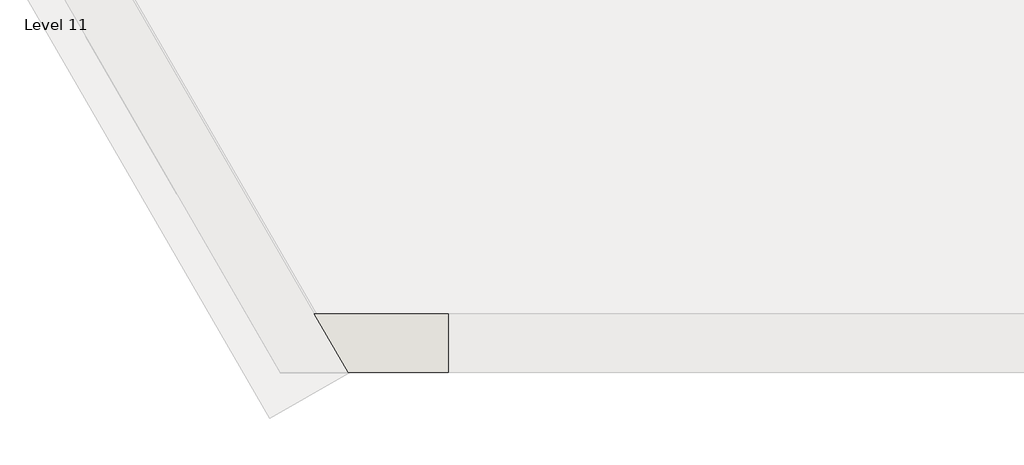
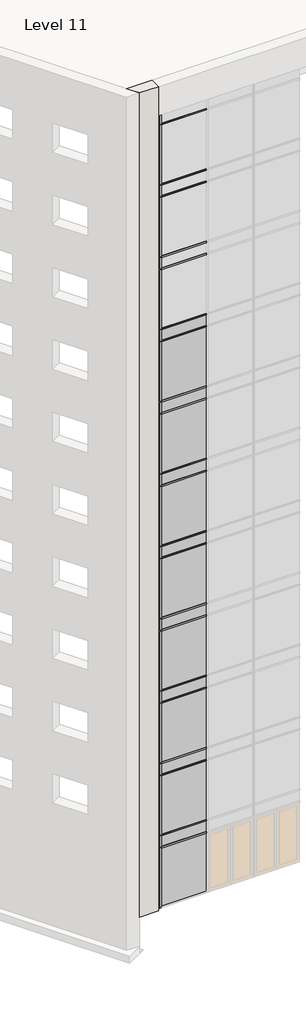
# One storey, part 1 of 6: 89 members, 38 plates, 1 wall.
"""IFC4 building model written with IfcOpenShell, lengths in millimetres."""

import ifcopenshell
import ifcopenshell.guid

model = None  # the IFC model being written
_history = None  # IfcOwnerHistory: only IFC2X3 demands one
_inside = {}  # id of a spatial element -> (the spatial element, [elements in it])
_under = {}  # id of a project, library or spatial element -> (it, [spatial elements below it])
_declared = {}  # id of a project -> (the project, [libraries it declares])
_typed = {}  # id of a type object -> (the type object, [elements of that type])
_made_of = {}  # id of a material, layer set ... -> (it, [elements and type objects made of it])


def new_model(schema):
    """Start an empty IFC model of exactly this schema.

    Asked for "IFC4X3", IfcOpenShell would pick the latest addendum, in which some entities
    have other attributes; the version numbers below select the first issue.
    IFC2X3 requires an IfcOwnerHistory on every rooted entity: one is made here for all.
    """
    global model, _history
    if schema == "IFC4X3":
        model = ifcopenshell.file(schema_version=(4, 3, 0, 0))
    else:
        model = ifcopenshell.file(schema=schema)
    _inside.clear()
    _under.clear()
    _declared.clear()
    _typed.clear()
    _made_of.clear()
    _history = None
    if model.schema == "IFC2X3":
        org = make("IfcOrganization", Name="unknown")
        user = make(
            "IfcPersonAndOrganization",
            ThePerson=make("IfcPerson", FamilyName="unknown"),
            TheOrganization=org,
        )
        app = make(
            "IfcApplication",
            ApplicationDeveloper=org,
            Version="unknown",
            ApplicationFullName="unknown",
            ApplicationIdentifier="unknown",
        )
        _history = make(
            "IfcOwnerHistory",
            OwningUser=user,
            OwningApplication=app,
            ChangeAction="ADDED",
            CreationDate=0,
        )
    return model


def make(cls, **values):
    """One entity of the class cls with the attributes given. An attribute that is None is left unset."""
    return model.create_entity(
        cls, **{name: value for name, value in values.items() if value is not None}
    )


def rooted(cls, **values):
    """An entity with a GlobalId (a new one), such as an element, a storey or a relation."""
    return make(cls, GlobalId=ifcopenshell.guid.new(), OwnerHistory=_history, **values)


def si_unit(unit_type, name, prefix=None):
    """IfcSIUnit, for example si_unit("LENGTHUNIT", "METRE", prefix="MILLI")."""
    return make("IfcSIUnit", UnitType=unit_type, Prefix=prefix, Name=name)


def assignment(units):
    """IfcUnitAssignment: the units of a project."""
    return None if units is None else make("IfcUnitAssignment", Units=units)


def point(xyz):
    """IfcCartesianPoint."""
    return None if xyz is None else make("IfcCartesianPoint", Coordinates=xyz)


def direction(xyz):
    """IfcDirection."""
    return None if xyz is None else make("IfcDirection", DirectionRatios=xyz)


def frame(location, z_axis=None, x_axis=None):
    """IfcAxis2Placement3D, a coordinate frame: its origin and axes. An axis left out is left unset."""
    return make(
        "IfcAxis2Placement3D",
        Location=point(location),
        Axis=direction(z_axis),
        RefDirection=direction(x_axis),
    )


def origin():
    """The frame at (0, 0, 0) with its axes left unset."""
    return frame((0.0, 0.0, 0.0))


def origin_with_axes():
    """The frame at (0, 0, 0) with the z axis (0, 0, 1) and the x axis (1, 0, 0) written out."""
    return frame((0.0, 0.0, 0.0), z_axis=(0.0, 0.0, 1.0), x_axis=(1.0, 0.0, 0.0))


def place(relative_to, where):
    """IfcLocalPlacement: puts the frame where relative to a parent placement (None: the world)."""
    return make(
        "IfcLocalPlacement", PlacementRelTo=relative_to, RelativePlacement=where
    )


def context(
    kind, dimensions, precision=None, world=None, true_north=None, identifier=None
):
    """IfcGeometricRepresentationContext, for example the 3D "Model" context."""
    return make(
        "IfcGeometricRepresentationContext",
        ContextIdentifier=identifier,
        ContextType=kind,
        CoordinateSpaceDimension=dimensions,
        Precision=precision,
        WorldCoordinateSystem=world,
        TrueNorth=true_north,
    )


def project(units=None, contexts=None):
    """IfcProject with its units and contexts."""
    return rooted(
        "IfcProject",
        Name="project",
        RepresentationContexts=contexts,
        UnitsInContext=assignment(units),
    )


def spatial(cls, under=None, at=None, **own):
    """A site, building, storey or space (cls), placed at a placement, below another one or the project."""
    s = rooted(cls, ObjectPlacement=at, **own)
    if under is not None:
        _under.setdefault(under.id(), (under, []))[1].append(s)
    return s


def polyline(points):
    """IfcPolyline through the points."""
    return make("IfcPolyline", Points=[point(p) for p in points])


def outline(outer, holes=None, kind="AREA"):
    """IfcArbitraryClosedProfileDef: a profile drawn as a closed curve; with holes, ...WithVoids."""
    if holes is None:
        return make("IfcArbitraryClosedProfileDef", ProfileType=kind, OuterCurve=outer)
    return make(
        "IfcArbitraryProfileDefWithVoids",
        ProfileType=kind,
        OuterCurve=outer,
        InnerCurves=holes,
    )


def extrude(swept, where, along, depth):
    """IfcExtrudedAreaSolid: the profile swept, set in the frame where, extruded along a direction by depth."""
    return make(
        "IfcExtrudedAreaSolid",
        SweptArea=swept,
        Position=where,
        ExtrudedDirection=direction(along),
        Depth=depth,
    )


def shape(context_of_items, identifier, shape_type, items):
    """IfcShapeRepresentation: the items that make up one representation, for example the "Body"."""
    return make(
        "IfcShapeRepresentation",
        ContextOfItems=context_of_items,
        RepresentationIdentifier=identifier,
        RepresentationType=shape_type,
        Items=items,
    )


def source(mapping_origin, context_of_items, identifier, shape_type, items):
    """IfcRepresentationMap: a shape defined once, which mapped items show again and again."""
    return make(
        "IfcRepresentationMap",
        MappingOrigin=mapping_origin,
        MappedRepresentation=shape(context_of_items, identifier, shape_type, items),
    )


def transform(
    local_origin,
    x_axis=None,
    y_axis=None,
    z_axis=None,
    scale=None,
    scale2=None,
    scale3=None,
    uniform=True,
):
    """IfcCartesianTransformationOperator3D, or its non-uniform kind. x_axis, y_axis, z_axis: its Axis1, 2, 3."""
    if uniform:
        return make(
            "IfcCartesianTransformationOperator3D",
            Axis1=direction(x_axis),
            Axis2=direction(y_axis),
            LocalOrigin=point(local_origin),
            Scale=scale,
            Axis3=direction(z_axis),
        )
    return make(
        "IfcCartesianTransformationOperator3DnonUniform",
        Axis1=direction(x_axis),
        Axis2=direction(y_axis),
        LocalOrigin=point(local_origin),
        Scale=scale,
        Axis3=direction(z_axis),
        Scale2=scale2,
        Scale3=scale3,
    )


def mapped(mapping_source, mapping_target):
    """IfcMappedItem: shows the shape of a source again, moved by a transform."""
    return make(
        "IfcMappedItem", MappingSource=mapping_source, MappingTarget=mapping_target
    )


def made_of(thing, what):
    """Note that an element or type object is made of a material, layer set ...; save() writes the relation."""
    if what is not None:
        _made_of.setdefault(what.id(), (what, []))[1].append(thing)
    return thing


def element(
    cls,
    number,
    at=None,
    inside=None,
    cuts=None,
    type_object=None,
    material=None,
    context=None,
    identifier="Body",
    shape_type=None,
    held_by="IfcProductDefinitionShape",
    body=None,
    shapes=None,
    **own,
):
    """One element of the class cls, such as IfcWall. Its Tag is "e" and its number.

    at: its placement. inside: the storey or other place that contains it. cuts: it is an
    opening in that element (IfcRelVoidsElement). A single representation is given by context,
    identifier, shape_type and body (its items); several are given by shapes. held_by: the class
    of the entity that holds the representations. save() writes the other relations.
    """
    e = rooted(cls, Tag="e%d" % number, ObjectPlacement=at, **own)
    if body is not None:
        shapes = [shape(context, identifier, shape_type, body)]
    if shapes is not None:
        e.Representation = make(held_by, Representations=shapes)
    if inside is not None:
        _inside.setdefault(inside.id(), (inside, []))[1].append(e)
    if cuts is not None:
        rooted(
            "IfcRelVoidsElement", RelatingBuildingElement=cuts, RelatedOpeningElement=e
        )
    if type_object is not None:
        _typed.setdefault(type_object.id(), (type_object, []))[1].append(e)
    return made_of(e, material)


def aggregate(whole, parts):
    """IfcRelAggregates: a whole, such as a stair, and the parts it consists of."""
    return rooted("IfcRelAggregates", RelatingObject=whole, RelatedObjects=parts)


def save(model, path):
    """Write the relations noted so far, then the file.

    IfcRelAggregates (storeys below a building ...), IfcRelContainedInSpatialStructure (elements
    in a storey), IfcRelDefinesByType, IfcRelAssociatesMaterial and IfcRelDeclares: one each for
    every whole, place, type object, material and project.
    """
    for whole, parts in _under.values():
        aggregate(whole, parts)
    for where, things in _inside.values():
        rooted(
            "IfcRelContainedInSpatialStructure",
            RelatedElements=things,
            RelatingStructure=where,
        )
    for kind, things in _typed.values():
        rooted("IfcRelDefinesByType", RelatedObjects=things, RelatingType=kind)
    for what, things in _made_of.values():
        rooted("IfcRelAssociatesMaterial", RelatedObjects=things, RelatingMaterial=what)
    for by, libraries in _declared.values():
        rooted("IfcRelDeclares", RelatingContext=by, RelatedDefinitions=libraries)
    model.write(path)


def rectangular_mullion_50x150mm_eb9201c3(model_context):
    return source(origin(), model_context, "Body", "SweptSolid", [
        extrude(outline(polyline([(25.0, 75.0), (25.0, -75.0), (-25.0, -75.0), (-25.0, 75.0), (25.0, 75.0)])), frame((0.0, 0.0, -2500.0), z_axis=(0.0, 0.0, 1.0), x_axis=(1.0, 0.0, 0.0)), (0.0, 0.0, 1.0), 2500.0),
    ])


def rectangular_mullion_50x150mm_f5b8645b(model_context):
    return source(origin(), model_context, "Body", "SweptSolid", [
        extrude(outline(polyline([(25.0, 75.0), (25.0, -75.0), (-25.0, -75.0), (-25.0, 75.0), (25.0, 75.0)])), frame((0.0, 0.0, -1780.0), z_axis=(0.0, 0.0, 1.0), x_axis=(1.0, 0.0, 0.0)), (0.0, 0.0, 1.0), 1780.0),
    ])


def rectangular_mullion_50x150mm_ded00a16(model_context):
    return source(origin(), model_context, "Body", "SweptSolid", [
        extrude(outline(polyline([(0.0, 75.0), (0.0, -75.0), (-50.0, -75.0), (-50.0, 75.0), (0.0, 75.0)])), frame((0.0, 0.0, -1780.0), z_axis=(0.0, 0.0, 1.0), x_axis=(1.0, 0.0, 0.0)), (0.0, 0.0, 1.0), 1780.0),
    ])


def rectangular_mullion_50x150mm_22f77a7a(model_context):
    return source(origin(), model_context, "Body", "SweptSolid", [
        extrude(outline(polyline([(25.0, 75.0), (25.0, -75.0), (-25.0, -75.0), (-25.0, 75.0), (25.0, 75.0)])), frame((0.0, 0.0, -500.0), z_axis=(0.0, 0.0, 1.0), x_axis=(1.0, 0.0, 0.0)), (0.0, 0.0, 1.0), 500.0),
    ])


def rectangular_mullion_50x150mm_4c3b9bdb(model_context):
    return source(origin(), model_context, "Body", "SweptSolid", [
        extrude(outline(polyline([(0.0, 75.0), (0.0, -75.0), (-50.0, -75.0), (-50.0, 75.0), (0.0, 75.0)])), frame((0.0, 0.0, -2500.0), z_axis=(0.0, 0.0, 1.0), x_axis=(1.0, 0.0, 0.0)), (0.0, 0.0, 1.0), 2500.0),
    ])


def rectangular_mullion_50x150mm_b3666dbd(model_context):
    return source(origin(), model_context, "Body", "SweptSolid", [
        extrude(outline(polyline([(0.0, 75.0), (0.0, -75.0), (-50.0, -75.0), (-50.0, 75.0), (0.0, 75.0)])), frame((0.0, 0.0, -500.0), z_axis=(0.0, 0.0, 1.0), x_axis=(1.0, 0.0, 0.0)), (0.0, 0.0, 1.0), 500.0),
    ])


def rectangular_mullion_50x150mm_6eefbde0(model_context):
    return source(origin(), model_context, "Body", "SweptSolid", [
        extrude(outline(polyline([(0.0, 75.0), (0.0, -75.0), (-50.0, -75.0), (-50.0, 75.0), (0.0, 75.0)])), frame((0.0, 0.0, -74.4185145), z_axis=(0.0, 0.0, 1.0), x_axis=(1.0, 0.0, 0.0)), (0.0, 0.0, 1.0), 74.4185145),
    ])


def rectangular_mullion_50x150mm_0166ad73(model_context):
    return source(origin(), model_context, "Body", "SweptSolid", [
        extrude(outline(polyline([(25.0, 75.0), (25.0, -75.0), (-25.0, -75.0), (-25.0, 75.0), (25.0, 75.0)])), frame((0.0, 0.0, -74.4185145), z_axis=(0.0, 0.0, 1.0), x_axis=(1.0, 0.0, 0.0)), (0.0, 0.0, 1.0), 74.4185145),
    ])


def system_panel_glazed_37b58b52(model_context):
    return source(origin(), model_context, "Body", "SweptSolid", [
        extrude(outline(polyline([(890.0, 24.5), (-890.0, 24.5), (-890.0, 49.5), (890.0, 49.5), (890.0, 24.5)])), origin_with_axes(), (0.0, 0.0, 1.0), 2425.0),
    ])


def system_panel_glazed_87c86ac8(model_context):
    return source(origin(), model_context, "Body", "SweptSolid", [
        extrude(outline(polyline([(890.0, 24.5), (-890.0, 24.5), (-890.0, 49.5), (890.0, 49.5), (890.0, 24.5)])), origin_with_axes(), (0.0, 0.0, 1.0), 450.0),
    ])


def system_panel_glazed_3dade0f0(model_context):
    return source(origin(), model_context, "Body", "SweptSolid", [
        extrude(outline(polyline([(890.0, 24.5), (-890.0, 24.5), (-890.0, 49.5), (890.0, 49.5), (890.0, 24.5)])), origin_with_axes(), (0.0, 0.0, 1.0), 2450.0),
    ])


def system_panel_glazed_e32ff5c7(model_context):
    return source(origin(), model_context, "Body", "SweptSolid", [
        extrude(outline(polyline([(37.2092572, 24.5), (-37.2092572, 24.5), (-37.2092572, 49.5), (37.2092572, 49.5), (37.2092572, 24.5)])), origin_with_axes(), (0.0, 0.0, 1.0), 2425.0),
    ])


def system_panel_glazed_b42e89e7(model_context):
    return source(origin(), model_context, "Body", "SweptSolid", [
        extrude(outline(polyline([(37.2092572, 24.5), (-37.2092572, 24.5), (-37.2092572, 49.5), (37.2092572, 49.5), (37.2092572, 24.5)])), origin_with_axes(), (0.0, 0.0, 1.0), 450.0),
    ])


def system_panel_glazed_54eb7814(model_context):
    return source(origin(), model_context, "Body", "SweptSolid", [
        extrude(outline(polyline([(37.2092572, 24.5), (-37.2092572, 24.5), (-37.2092572, 49.5), (37.2092572, 49.5), (37.2092572, 24.5)])), origin_with_axes(), (0.0, 0.0, 1.0), 2450.0),
    ])


def system_panel_glazed_e987ce54(model_context):
    return source(origin(), model_context, "Body", "SweptSolid", [
        extrude(outline(polyline([(37.2092572, 24.5), (-37.2092572, 24.5), (-37.2092572, 49.5), (37.2092572, 49.5), (37.2092572, 24.5)])), origin_with_axes(), (0.0, 0.0, 1.0), 425.0),
    ])


model = new_model("IFC4")

# Units and contexts
model_context = context("Model", 3, world=origin())
ifc_project = project(units=[si_unit("LENGTHUNIT", "METRE", prefix="MILLI")], contexts=[model_context])

# Site, building, storey
site = spatial("IfcSite", under=ifc_project)
building = spatial("IfcBuilding", under=site)
storey = spatial("IfcBuildingStorey", under=building, Name="Level 11", Elevation=33000.0)

# Members
placement = place(None, origin())
rectangular_mullion_50x150mm_shape = rectangular_mullion_50x150mm_eb9201c3(model_context)
element("IfcMember", 1, ObjectType="Rectangular Mullion : 50x150mm", at=placement, inside=storey, context=model_context, shape_type="MappedRepresentation", body=[
    mapped(rectangular_mullion_50x150mm_shape, transform((-3631.4360441, -8316.0631989, 0.0), x_axis=(-1.0, 0.0, 0.0), y_axis=(0.0, 1.0, 0.0), z_axis=(0.0, 0.0, -1.0))),
])
rectangular_mullion_50x150mm_2_shape = rectangular_mullion_50x150mm_f5b8645b(model_context)
element("IfcMember", 2, ObjectType="Rectangular Mullion : 50x150mm", at=placement, inside=storey, context=model_context, shape_type="MappedRepresentation", body=[
    mapped(rectangular_mullion_50x150mm_2_shape, transform((-3606.4360441, -8316.0631989, 2500.0), x_axis=(0.0, 0.0, 1.0), y_axis=(0.0, 1.0, 0.0), z_axis=(-1.0, 0.0, 0.0))),
])
element("IfcMember", 3, ObjectType="Rectangular Mullion : 50x150mm", at=placement, inside=storey, context=model_context, shape_type="MappedRepresentation", body=[
    mapped(rectangular_mullion_50x150mm_2_shape, transform((-3606.4360441, -8316.0631989, 5500.0), x_axis=(0.0, 0.0, 1.0), y_axis=(0.0, 1.0, 0.0), z_axis=(-1.0, 0.0, 0.0))),
])
element("IfcMember", 4, ObjectType="Rectangular Mullion : 50x150mm", at=placement, inside=storey, context=model_context, shape_type="MappedRepresentation", body=[
    mapped(rectangular_mullion_50x150mm_2_shape, transform((-3606.4360441, -8316.0631989, 8500.0), x_axis=(0.0, 0.0, 1.0), y_axis=(0.0, 1.0, 0.0), z_axis=(-1.0, 0.0, 0.0))),
])
element("IfcMember", 5, ObjectType="Rectangular Mullion : 50x150mm", at=placement, inside=storey, context=model_context, shape_type="MappedRepresentation", body=[
    mapped(rectangular_mullion_50x150mm_2_shape, transform((-3606.4360441, -8316.0631989, 11500.0), x_axis=(0.0, 0.0, 1.0), y_axis=(0.0, 1.0, 0.0), z_axis=(-1.0, 0.0, 0.0))),
])
element("IfcMember", 6, ObjectType="Rectangular Mullion : 50x150mm", at=placement, inside=storey, context=model_context, shape_type="MappedRepresentation", body=[
    mapped(rectangular_mullion_50x150mm_2_shape, transform((-3606.4360441, -8316.0631989, 14500.0), x_axis=(0.0, 0.0, 1.0), y_axis=(0.0, 1.0, 0.0), z_axis=(-1.0, 0.0, 0.0))),
])
element("IfcMember", 7, ObjectType="Rectangular Mullion : 50x150mm", at=placement, inside=storey, context=model_context, shape_type="MappedRepresentation", body=[
    mapped(rectangular_mullion_50x150mm_2_shape, transform((-3606.4360441, -8316.0631989, 17500.0), x_axis=(0.0, 0.0, 1.0), y_axis=(0.0, 1.0, 0.0), z_axis=(-1.0, 0.0, 0.0))),
])
element("IfcMember", 8, ObjectType="Rectangular Mullion : 50x150mm", at=placement, inside=storey, context=model_context, shape_type="MappedRepresentation", body=[
    mapped(rectangular_mullion_50x150mm_2_shape, transform((-3606.4360441, -8316.0631989, 20500.0), x_axis=(0.0, 0.0, 1.0), y_axis=(0.0, 1.0, 0.0), z_axis=(-1.0, 0.0, 0.0))),
])
element("IfcMember", 9, ObjectType="Rectangular Mullion : 50x150mm", at=placement, inside=storey, context=model_context, shape_type="MappedRepresentation", body=[
    mapped(rectangular_mullion_50x150mm_2_shape, transform((-3606.4360441, -8316.0631989, 23500.0), x_axis=(0.0, 0.0, 1.0), y_axis=(0.0, 1.0, 0.0), z_axis=(-1.0, 0.0, 0.0))),
])
element("IfcMember", 10, ObjectType="Rectangular Mullion : 50x150mm", at=placement, inside=storey, context=model_context, shape_type="MappedRepresentation", body=[
    mapped(rectangular_mullion_50x150mm_2_shape, transform((-3606.4360441, -8316.0631989, 3000.0), x_axis=(0.0, 0.0, 1.0), y_axis=(0.0, 1.0, 0.0), z_axis=(-1.0, 0.0, 0.0))),
])
element("IfcMember", 11, ObjectType="Rectangular Mullion : 50x150mm", at=placement, inside=storey, context=model_context, shape_type="MappedRepresentation", body=[
    mapped(rectangular_mullion_50x150mm_2_shape, transform((-3606.4360441, -8316.0631989, 6000.0), x_axis=(0.0, 0.0, 1.0), y_axis=(0.0, 1.0, 0.0), z_axis=(-1.0, 0.0, 0.0))),
])
element("IfcMember", 12, ObjectType="Rectangular Mullion : 50x150mm", at=placement, inside=storey, context=model_context, shape_type="MappedRepresentation", body=[
    mapped(rectangular_mullion_50x150mm_2_shape, transform((-3606.4360441, -8316.0631989, 9000.0), x_axis=(0.0, 0.0, 1.0), y_axis=(0.0, 1.0, 0.0), z_axis=(-1.0, 0.0, 0.0))),
])
element("IfcMember", 13, ObjectType="Rectangular Mullion : 50x150mm", at=placement, inside=storey, context=model_context, shape_type="MappedRepresentation", body=[
    mapped(rectangular_mullion_50x150mm_2_shape, transform((-3606.4360441, -8316.0631989, 12000.0), x_axis=(0.0, 0.0, 1.0), y_axis=(0.0, 1.0, 0.0), z_axis=(-1.0, 0.0, 0.0))),
])
element("IfcMember", 14, ObjectType="Rectangular Mullion : 50x150mm", at=placement, inside=storey, context=model_context, shape_type="MappedRepresentation", body=[
    mapped(rectangular_mullion_50x150mm_2_shape, transform((-3606.4360441, -8316.0631989, 15000.0), x_axis=(0.0, 0.0, 1.0), y_axis=(0.0, 1.0, 0.0), z_axis=(-1.0, 0.0, 0.0))),
])
element("IfcMember", 15, ObjectType="Rectangular Mullion : 50x150mm", at=placement, inside=storey, context=model_context, shape_type="MappedRepresentation", body=[
    mapped(rectangular_mullion_50x150mm_2_shape, transform((-3606.4360441, -8316.0631989, 18000.0), x_axis=(0.0, 0.0, 1.0), y_axis=(0.0, 1.0, 0.0), z_axis=(-1.0, 0.0, 0.0))),
])
element("IfcMember", 16, ObjectType="Rectangular Mullion : 50x150mm", at=placement, inside=storey, context=model_context, shape_type="MappedRepresentation", body=[
    mapped(rectangular_mullion_50x150mm_2_shape, transform((-3606.4360441, -8316.0631989, 21000.0), x_axis=(0.0, 0.0, 1.0), y_axis=(0.0, 1.0, 0.0), z_axis=(-1.0, 0.0, 0.0))),
])
element("IfcMember", 17, ObjectType="Rectangular Mullion : 50x150mm", at=placement, inside=storey, context=model_context, shape_type="MappedRepresentation", body=[
    mapped(rectangular_mullion_50x150mm_2_shape, transform((-3606.4360441, -8316.0631989, 24000.0), x_axis=(0.0, 0.0, 1.0), y_axis=(0.0, 1.0, 0.0), z_axis=(-1.0, 0.0, 0.0))),
])
element("IfcMember", 18, ObjectType="Rectangular Mullion : 50x150mm", at=placement, inside=storey, context=model_context, shape_type="MappedRepresentation", body=[
    mapped(rectangular_mullion_50x150mm_2_shape, transform((-3606.4360441, -8316.0631989, 27000.0), x_axis=(0.0, 0.0, 1.0), y_axis=(0.0, 1.0, 0.0), z_axis=(-1.0, 0.0, 0.0))),
])
element("IfcMember", 19, ObjectType="Rectangular Mullion : 50x150mm", at=placement, inside=storey, context=model_context, shape_type="MappedRepresentation", body=[
    mapped(rectangular_mullion_50x150mm_2_shape, transform((-3606.4360441, -8316.0631989, 26500.0), x_axis=(0.0, 0.0, 1.0), y_axis=(0.0, 1.0, 0.0), z_axis=(-1.0, 0.0, 0.0))),
])
element("IfcMember", 20, ObjectType="Rectangular Mullion : 50x150mm", at=placement, inside=storey, context=model_context, shape_type="MappedRepresentation", body=[
    mapped(rectangular_mullion_50x150mm_2_shape, transform((-3606.4360441, -8316.0631989, 30000.0), x_axis=(0.0, 0.0, 1.0), y_axis=(0.0, 1.0, 0.0), z_axis=(-1.0, 0.0, 0.0))),
])
element("IfcMember", 21, ObjectType="Rectangular Mullion : 50x150mm", at=placement, inside=storey, context=model_context, shape_type="MappedRepresentation", body=[
    mapped(rectangular_mullion_50x150mm_2_shape, transform((-3606.4360441, -8316.0631989, 29500.0), x_axis=(0.0, 0.0, 1.0), y_axis=(0.0, 1.0, 0.0), z_axis=(-1.0, 0.0, 0.0))),
])
element("IfcMember", 22, ObjectType="Rectangular Mullion : 50x150mm", at=placement, inside=storey, context=model_context, shape_type="MappedRepresentation", body=[
    mapped(rectangular_mullion_50x150mm_2_shape, transform((-3606.4360441, -8316.0631989, 32500.0), x_axis=(0.0, 0.0, 1.0), y_axis=(0.0, 1.0, 0.0), z_axis=(-1.0, 0.0, 0.0))),
])
rectangular_mullion_50x150mm_3_shape = rectangular_mullion_50x150mm_ded00a16(model_context)
element("IfcMember", 23, ObjectType="Rectangular Mullion : 50x150mm", at=placement, inside=storey, context=model_context, shape_type="MappedRepresentation", body=[
    mapped(rectangular_mullion_50x150mm_3_shape, transform((-3606.4360441, -8316.0631989, 33000.0), x_axis=(0.0, 0.0, 1.0), y_axis=(0.0, 1.0, 0.0), z_axis=(-1.0, 0.0, 0.0))),
])
rectangular_mullion_50x150mm_4_shape = rectangular_mullion_50x150mm_22f77a7a(model_context)
element("IfcMember", 24, ObjectType="Rectangular Mullion : 50x150mm", at=placement, inside=storey, context=model_context, shape_type="MappedRepresentation", body=[
    mapped(rectangular_mullion_50x150mm_4_shape, transform((-3631.4360441, -8316.0631989, 2500.0), x_axis=(-1.0, 0.0, 0.0), y_axis=(0.0, 1.0, 0.0), z_axis=(0.0, 0.0, -1.0))),
])
element("IfcMember", 25, ObjectType="Rectangular Mullion : 50x150mm", at=placement, inside=storey, context=model_context, shape_type="MappedRepresentation", body=[
    mapped(rectangular_mullion_50x150mm_4_shape, transform((-3631.4360441, -8316.0631989, 5500.0), x_axis=(-1.0, 0.0, 0.0), y_axis=(0.0, 1.0, 0.0), z_axis=(0.0, 0.0, -1.0))),
])
element("IfcMember", 26, ObjectType="Rectangular Mullion : 50x150mm", at=placement, inside=storey, context=model_context, shape_type="MappedRepresentation", body=[
    mapped(rectangular_mullion_50x150mm_4_shape, transform((-3631.4360441, -8316.0631989, 8500.0), x_axis=(-1.0, 0.0, 0.0), y_axis=(0.0, 1.0, 0.0), z_axis=(0.0, 0.0, -1.0))),
])
element("IfcMember", 27, ObjectType="Rectangular Mullion : 50x150mm", at=placement, inside=storey, context=model_context, shape_type="MappedRepresentation", body=[
    mapped(rectangular_mullion_50x150mm_4_shape, transform((-3631.4360441, -8316.0631989, 11500.0), x_axis=(-1.0, 0.0, 0.0), y_axis=(0.0, 1.0, 0.0), z_axis=(0.0, 0.0, -1.0))),
])
element("IfcMember", 28, ObjectType="Rectangular Mullion : 50x150mm", at=placement, inside=storey, context=model_context, shape_type="MappedRepresentation", body=[
    mapped(rectangular_mullion_50x150mm_4_shape, transform((-3631.4360441, -8316.0631989, 14500.0), x_axis=(-1.0, 0.0, 0.0), y_axis=(0.0, 1.0, 0.0), z_axis=(0.0, 0.0, -1.0))),
])
element("IfcMember", 29, ObjectType="Rectangular Mullion : 50x150mm", at=placement, inside=storey, context=model_context, shape_type="MappedRepresentation", body=[
    mapped(rectangular_mullion_50x150mm_4_shape, transform((-3631.4360441, -8316.0631989, 17500.0), x_axis=(-1.0, 0.0, 0.0), y_axis=(0.0, 1.0, 0.0), z_axis=(0.0, 0.0, -1.0))),
])
element("IfcMember", 30, ObjectType="Rectangular Mullion : 50x150mm", at=placement, inside=storey, context=model_context, shape_type="MappedRepresentation", body=[
    mapped(rectangular_mullion_50x150mm_4_shape, transform((-3631.4360441, -8316.0631989, 20500.0), x_axis=(-1.0, 0.0, 0.0), y_axis=(0.0, 1.0, 0.0), z_axis=(0.0, 0.0, -1.0))),
])
element("IfcMember", 31, ObjectType="Rectangular Mullion : 50x150mm", at=placement, inside=storey, context=model_context, shape_type="MappedRepresentation", body=[
    mapped(rectangular_mullion_50x150mm_4_shape, transform((-3631.4360441, -8316.0631989, 23500.0), x_axis=(-1.0, 0.0, 0.0), y_axis=(0.0, 1.0, 0.0), z_axis=(0.0, 0.0, -1.0))),
])
element("IfcMember", 32, ObjectType="Rectangular Mullion : 50x150mm", at=placement, inside=storey, context=model_context, shape_type="MappedRepresentation", body=[
    mapped(rectangular_mullion_50x150mm_4_shape, transform((-3631.4360441, -8316.0631989, 26500.0), x_axis=(-1.0, 0.0, 0.0), y_axis=(0.0, 1.0, 0.0), z_axis=(0.0, 0.0, -1.0))),
])
element("IfcMember", 33, ObjectType="Rectangular Mullion : 50x150mm", at=placement, inside=storey, context=model_context, shape_type="MappedRepresentation", body=[
    mapped(rectangular_mullion_50x150mm_4_shape, transform((-3631.4360441, -8316.0631989, 29500.0), x_axis=(-1.0, 0.0, 0.0), y_axis=(0.0, 1.0, 0.0), z_axis=(0.0, 0.0, -1.0))),
])
element("IfcMember", 34, ObjectType="Rectangular Mullion : 50x150mm", at=placement, inside=storey, context=model_context, shape_type="MappedRepresentation", body=[
    mapped(rectangular_mullion_50x150mm_shape, transform((-3631.4360441, -8316.0631989, 3000.0), x_axis=(-1.0, 0.0, 0.0), y_axis=(0.0, 1.0, 0.0), z_axis=(0.0, 0.0, -1.0))),
])
element("IfcMember", 35, ObjectType="Rectangular Mullion : 50x150mm", at=placement, inside=storey, context=model_context, shape_type="MappedRepresentation", body=[
    mapped(rectangular_mullion_50x150mm_shape, transform((-3631.4360441, -8316.0631989, 6000.0), x_axis=(-1.0, 0.0, 0.0), y_axis=(0.0, 1.0, 0.0), z_axis=(0.0, 0.0, -1.0))),
])
element("IfcMember", 36, ObjectType="Rectangular Mullion : 50x150mm", at=placement, inside=storey, context=model_context, shape_type="MappedRepresentation", body=[
    mapped(rectangular_mullion_50x150mm_shape, transform((-3631.4360441, -8316.0631989, 9000.0), x_axis=(-1.0, 0.0, 0.0), y_axis=(0.0, 1.0, 0.0), z_axis=(0.0, 0.0, -1.0))),
])
element("IfcMember", 37, ObjectType="Rectangular Mullion : 50x150mm", at=placement, inside=storey, context=model_context, shape_type="MappedRepresentation", body=[
    mapped(rectangular_mullion_50x150mm_shape, transform((-3631.4360441, -8316.0631989, 12000.0), x_axis=(-1.0, 0.0, 0.0), y_axis=(0.0, 1.0, 0.0), z_axis=(0.0, 0.0, -1.0))),
])
element("IfcMember", 38, ObjectType="Rectangular Mullion : 50x150mm", at=placement, inside=storey, context=model_context, shape_type="MappedRepresentation", body=[
    mapped(rectangular_mullion_50x150mm_shape, transform((-3631.4360441, -8316.0631989, 15000.0), x_axis=(-1.0, 0.0, 0.0), y_axis=(0.0, 1.0, 0.0), z_axis=(0.0, 0.0, -1.0))),
])
element("IfcMember", 39, ObjectType="Rectangular Mullion : 50x150mm", at=placement, inside=storey, context=model_context, shape_type="MappedRepresentation", body=[
    mapped(rectangular_mullion_50x150mm_shape, transform((-3631.4360441, -8316.0631989, 18000.0), x_axis=(-1.0, 0.0, 0.0), y_axis=(0.0, 1.0, 0.0), z_axis=(0.0, 0.0, -1.0))),
])
element("IfcMember", 40, ObjectType="Rectangular Mullion : 50x150mm", at=placement, inside=storey, context=model_context, shape_type="MappedRepresentation", body=[
    mapped(rectangular_mullion_50x150mm_shape, transform((-3631.4360441, -8316.0631989, 21000.0), x_axis=(-1.0, 0.0, 0.0), y_axis=(0.0, 1.0, 0.0), z_axis=(0.0, 0.0, -1.0))),
])
element("IfcMember", 41, ObjectType="Rectangular Mullion : 50x150mm", at=placement, inside=storey, context=model_context, shape_type="MappedRepresentation", body=[
    mapped(rectangular_mullion_50x150mm_shape, transform((-3631.4360441, -8316.0631989, 24000.0), x_axis=(-1.0, 0.0, 0.0), y_axis=(0.0, 1.0, 0.0), z_axis=(0.0, 0.0, -1.0))),
])
element("IfcMember", 42, ObjectType="Rectangular Mullion : 50x150mm", at=placement, inside=storey, context=model_context, shape_type="MappedRepresentation", body=[
    mapped(rectangular_mullion_50x150mm_shape, transform((-3631.4360441, -8316.0631989, 27000.0), x_axis=(-1.0, 0.0, 0.0), y_axis=(0.0, 1.0, 0.0), z_axis=(0.0, 0.0, -1.0))),
])
element("IfcMember", 43, ObjectType="Rectangular Mullion : 50x150mm", at=placement, inside=storey, context=model_context, shape_type="MappedRepresentation", body=[
    mapped(rectangular_mullion_50x150mm_shape, transform((-3631.4360441, -8316.0631989, 30000.0), x_axis=(-1.0, 0.0, 0.0), y_axis=(0.0, 1.0, 0.0), z_axis=(0.0, 0.0, -1.0))),
])
element("IfcMember", 44, ObjectType="Rectangular Mullion : 50x150mm", at=placement, inside=storey, context=model_context, shape_type="MappedRepresentation", body=[
    mapped(rectangular_mullion_50x150mm_4_shape, transform((-3631.4360441, -8316.0631989, 32500.0), x_axis=(-1.0, 0.0, 0.0), y_axis=(0.0, 1.0, 0.0), z_axis=(0.0, 0.0, -1.0))),
])
rectangular_mullion_50x150mm_5_shape = rectangular_mullion_50x150mm_4c3b9bdb(model_context)
element("IfcMember", 45, ObjectType="Rectangular Mullion : 50x150mm", at=placement, inside=storey, context=model_context, shape_type="MappedRepresentation", body=[
    mapped(rectangular_mullion_50x150mm_5_shape, transform((-3780.8545586, -8316.0631989, 0.0), x_axis=(-1.0, 0.0, 0.0), y_axis=(0.0, 1.0, 0.0), z_axis=(0.0, 0.0, -1.0))),
])
rectangular_mullion_50x150mm_6_shape = rectangular_mullion_50x150mm_b3666dbd(model_context)
element("IfcMember", 46, ObjectType="Rectangular Mullion : 50x150mm", at=placement, inside=storey, context=model_context, shape_type="MappedRepresentation", body=[
    mapped(rectangular_mullion_50x150mm_6_shape, transform((-3780.8545586, -8316.0631989, 2500.0), x_axis=(-1.0, 0.0, 0.0), y_axis=(0.0, 1.0, 0.0), z_axis=(0.0, 0.0, -1.0))),
])
element("IfcMember", 47, ObjectType="Rectangular Mullion : 50x150mm", at=placement, inside=storey, context=model_context, shape_type="MappedRepresentation", body=[
    mapped(rectangular_mullion_50x150mm_6_shape, transform((-3780.8545586, -8316.0631989, 5500.0), x_axis=(-1.0, 0.0, 0.0), y_axis=(0.0, 1.0, 0.0), z_axis=(0.0, 0.0, -1.0))),
])
element("IfcMember", 48, ObjectType="Rectangular Mullion : 50x150mm", at=placement, inside=storey, context=model_context, shape_type="MappedRepresentation", body=[
    mapped(rectangular_mullion_50x150mm_6_shape, transform((-3780.8545586, -8316.0631989, 8500.0), x_axis=(-1.0, 0.0, 0.0), y_axis=(0.0, 1.0, 0.0), z_axis=(0.0, 0.0, -1.0))),
])
element("IfcMember", 49, ObjectType="Rectangular Mullion : 50x150mm", at=placement, inside=storey, context=model_context, shape_type="MappedRepresentation", body=[
    mapped(rectangular_mullion_50x150mm_6_shape, transform((-3780.8545586, -8316.0631989, 11500.0), x_axis=(-1.0, 0.0, 0.0), y_axis=(0.0, 1.0, 0.0), z_axis=(0.0, 0.0, -1.0))),
])
element("IfcMember", 50, ObjectType="Rectangular Mullion : 50x150mm", at=placement, inside=storey, context=model_context, shape_type="MappedRepresentation", body=[
    mapped(rectangular_mullion_50x150mm_6_shape, transform((-3780.8545586, -8316.0631989, 14500.0), x_axis=(-1.0, 0.0, 0.0), y_axis=(0.0, 1.0, 0.0), z_axis=(0.0, 0.0, -1.0))),
])
element("IfcMember", 51, ObjectType="Rectangular Mullion : 50x150mm", at=placement, inside=storey, context=model_context, shape_type="MappedRepresentation", body=[
    mapped(rectangular_mullion_50x150mm_6_shape, transform((-3780.8545586, -8316.0631989, 17500.0), x_axis=(-1.0, 0.0, 0.0), y_axis=(0.0, 1.0, 0.0), z_axis=(0.0, 0.0, -1.0))),
])
element("IfcMember", 52, ObjectType="Rectangular Mullion : 50x150mm", at=placement, inside=storey, context=model_context, shape_type="MappedRepresentation", body=[
    mapped(rectangular_mullion_50x150mm_6_shape, transform((-3780.8545586, -8316.0631989, 20500.0), x_axis=(-1.0, 0.0, 0.0), y_axis=(0.0, 1.0, 0.0), z_axis=(0.0, 0.0, -1.0))),
])
element("IfcMember", 53, ObjectType="Rectangular Mullion : 50x150mm", at=placement, inside=storey, context=model_context, shape_type="MappedRepresentation", body=[
    mapped(rectangular_mullion_50x150mm_6_shape, transform((-3780.8545586, -8316.0631989, 23500.0), x_axis=(-1.0, 0.0, 0.0), y_axis=(0.0, 1.0, 0.0), z_axis=(0.0, 0.0, -1.0))),
])
element("IfcMember", 54, ObjectType="Rectangular Mullion : 50x150mm", at=placement, inside=storey, context=model_context, shape_type="MappedRepresentation", body=[
    mapped(rectangular_mullion_50x150mm_6_shape, transform((-3780.8545586, -8316.0631989, 26500.0), x_axis=(-1.0, 0.0, 0.0), y_axis=(0.0, 1.0, 0.0), z_axis=(0.0, 0.0, -1.0))),
])
element("IfcMember", 55, ObjectType="Rectangular Mullion : 50x150mm", at=placement, inside=storey, context=model_context, shape_type="MappedRepresentation", body=[
    mapped(rectangular_mullion_50x150mm_6_shape, transform((-3780.8545586, -8316.0631989, 29500.0), x_axis=(-1.0, 0.0, 0.0), y_axis=(0.0, 1.0, 0.0), z_axis=(0.0, 0.0, -1.0))),
])
element("IfcMember", 56, ObjectType="Rectangular Mullion : 50x150mm", at=placement, inside=storey, context=model_context, shape_type="MappedRepresentation", body=[
    mapped(rectangular_mullion_50x150mm_5_shape, transform((-3780.8545586, -8316.0631989, 3000.0), x_axis=(-1.0, 0.0, 0.0), y_axis=(0.0, 1.0, 0.0), z_axis=(0.0, 0.0, -1.0))),
])
element("IfcMember", 57, ObjectType="Rectangular Mullion : 50x150mm", at=placement, inside=storey, context=model_context, shape_type="MappedRepresentation", body=[
    mapped(rectangular_mullion_50x150mm_5_shape, transform((-3780.8545586, -8316.0631989, 6000.0), x_axis=(-1.0, 0.0, 0.0), y_axis=(0.0, 1.0, 0.0), z_axis=(0.0, 0.0, -1.0))),
])
element("IfcMember", 58, ObjectType="Rectangular Mullion : 50x150mm", at=placement, inside=storey, context=model_context, shape_type="MappedRepresentation", body=[
    mapped(rectangular_mullion_50x150mm_5_shape, transform((-3780.8545586, -8316.0631989, 9000.0), x_axis=(-1.0, 0.0, 0.0), y_axis=(0.0, 1.0, 0.0), z_axis=(0.0, 0.0, -1.0))),
])
element("IfcMember", 59, ObjectType="Rectangular Mullion : 50x150mm", at=placement, inside=storey, context=model_context, shape_type="MappedRepresentation", body=[
    mapped(rectangular_mullion_50x150mm_5_shape, transform((-3780.8545586, -8316.0631989, 12000.0), x_axis=(-1.0, 0.0, 0.0), y_axis=(0.0, 1.0, 0.0), z_axis=(0.0, 0.0, -1.0))),
])
element("IfcMember", 60, ObjectType="Rectangular Mullion : 50x150mm", at=placement, inside=storey, context=model_context, shape_type="MappedRepresentation", body=[
    mapped(rectangular_mullion_50x150mm_5_shape, transform((-3780.8545586, -8316.0631989, 15000.0), x_axis=(-1.0, 0.0, 0.0), y_axis=(0.0, 1.0, 0.0), z_axis=(0.0, 0.0, -1.0))),
])
element("IfcMember", 61, ObjectType="Rectangular Mullion : 50x150mm", at=placement, inside=storey, context=model_context, shape_type="MappedRepresentation", body=[
    mapped(rectangular_mullion_50x150mm_5_shape, transform((-3780.8545586, -8316.0631989, 18000.0), x_axis=(-1.0, 0.0, 0.0), y_axis=(0.0, 1.0, 0.0), z_axis=(0.0, 0.0, -1.0))),
])
element("IfcMember", 62, ObjectType="Rectangular Mullion : 50x150mm", at=placement, inside=storey, context=model_context, shape_type="MappedRepresentation", body=[
    mapped(rectangular_mullion_50x150mm_5_shape, transform((-3780.8545586, -8316.0631989, 21000.0), x_axis=(-1.0, 0.0, 0.0), y_axis=(0.0, 1.0, 0.0), z_axis=(0.0, 0.0, -1.0))),
])
element("IfcMember", 63, ObjectType="Rectangular Mullion : 50x150mm", at=placement, inside=storey, context=model_context, shape_type="MappedRepresentation", body=[
    mapped(rectangular_mullion_50x150mm_5_shape, transform((-3780.8545586, -8316.0631989, 24000.0), x_axis=(-1.0, 0.0, 0.0), y_axis=(0.0, 1.0, 0.0), z_axis=(0.0, 0.0, -1.0))),
])
element("IfcMember", 64, ObjectType="Rectangular Mullion : 50x150mm", at=placement, inside=storey, context=model_context, shape_type="MappedRepresentation", body=[
    mapped(rectangular_mullion_50x150mm_5_shape, transform((-3780.8545586, -8316.0631989, 27000.0), x_axis=(-1.0, 0.0, 0.0), y_axis=(0.0, 1.0, 0.0), z_axis=(0.0, 0.0, -1.0))),
])
element("IfcMember", 65, ObjectType="Rectangular Mullion : 50x150mm", at=placement, inside=storey, context=model_context, shape_type="MappedRepresentation", body=[
    mapped(rectangular_mullion_50x150mm_5_shape, transform((-3780.8545586, -8316.0631989, 30000.0), x_axis=(-1.0, 0.0, 0.0), y_axis=(0.0, 1.0, 0.0), z_axis=(0.0, 0.0, -1.0))),
])
element("IfcMember", 66, ObjectType="Rectangular Mullion : 50x150mm", at=placement, inside=storey, context=model_context, shape_type="MappedRepresentation", body=[
    mapped(rectangular_mullion_50x150mm_6_shape, transform((-3780.8545586, -8316.0631989, 32500.0), x_axis=(-1.0, 0.0, 0.0), y_axis=(0.0, 1.0, 0.0), z_axis=(0.0, 0.0, -1.0))),
])
rectangular_mullion_50x150mm_7_shape = rectangular_mullion_50x150mm_6eefbde0(model_context)
element("IfcMember", 67, ObjectType="Rectangular Mullion : 50x150mm", at=placement, inside=storey, context=model_context, shape_type="MappedRepresentation", body=[
    mapped(rectangular_mullion_50x150mm_7_shape, transform((-3730.8545586, -8316.0631989, 33000.0), x_axis=(0.0, 0.0, 1.0), y_axis=(0.0, 1.0, 0.0), z_axis=(-1.0, 0.0, 0.0))),
])
rectangular_mullion_50x150mm_8_shape = rectangular_mullion_50x150mm_0166ad73(model_context)
element("IfcMember", 68, ObjectType="Rectangular Mullion : 50x150mm", at=placement, inside=storey, context=model_context, shape_type="MappedRepresentation", body=[
    mapped(rectangular_mullion_50x150mm_8_shape, transform((-3730.8545586, -8316.0631989, 2500.0), x_axis=(0.0, 0.0, 1.0), y_axis=(0.0, 1.0, 0.0), z_axis=(-1.0, 0.0, 0.0))),
])
element("IfcMember", 69, ObjectType="Rectangular Mullion : 50x150mm", at=placement, inside=storey, context=model_context, shape_type="MappedRepresentation", body=[
    mapped(rectangular_mullion_50x150mm_8_shape, transform((-3730.8545586, -8316.0631989, 5500.0), x_axis=(0.0, 0.0, 1.0), y_axis=(0.0, 1.0, 0.0), z_axis=(-1.0, 0.0, 0.0))),
])
element("IfcMember", 70, ObjectType="Rectangular Mullion : 50x150mm", at=placement, inside=storey, context=model_context, shape_type="MappedRepresentation", body=[
    mapped(rectangular_mullion_50x150mm_8_shape, transform((-3730.8545586, -8316.0631989, 8500.0), x_axis=(0.0, 0.0, 1.0), y_axis=(0.0, 1.0, 0.0), z_axis=(-1.0, 0.0, 0.0))),
])
element("IfcMember", 71, ObjectType="Rectangular Mullion : 50x150mm", at=placement, inside=storey, context=model_context, shape_type="MappedRepresentation", body=[
    mapped(rectangular_mullion_50x150mm_8_shape, transform((-3730.8545586, -8316.0631989, 11500.0), x_axis=(0.0, 0.0, 1.0), y_axis=(0.0, 1.0, 0.0), z_axis=(-1.0, 0.0, 0.0))),
])
element("IfcMember", 72, ObjectType="Rectangular Mullion : 50x150mm", at=placement, inside=storey, context=model_context, shape_type="MappedRepresentation", body=[
    mapped(rectangular_mullion_50x150mm_8_shape, transform((-3730.8545586, -8316.0631989, 14500.0), x_axis=(0.0, 0.0, 1.0), y_axis=(0.0, 1.0, 0.0), z_axis=(-1.0, 0.0, 0.0))),
])
element("IfcMember", 73, ObjectType="Rectangular Mullion : 50x150mm", at=placement, inside=storey, context=model_context, shape_type="MappedRepresentation", body=[
    mapped(rectangular_mullion_50x150mm_8_shape, transform((-3730.8545586, -8316.0631989, 17500.0), x_axis=(0.0, 0.0, 1.0), y_axis=(0.0, 1.0, 0.0), z_axis=(-1.0, 0.0, 0.0))),
])
element("IfcMember", 74, ObjectType="Rectangular Mullion : 50x150mm", at=placement, inside=storey, context=model_context, shape_type="MappedRepresentation", body=[
    mapped(rectangular_mullion_50x150mm_8_shape, transform((-3730.8545586, -8316.0631989, 20500.0), x_axis=(0.0, 0.0, 1.0), y_axis=(0.0, 1.0, 0.0), z_axis=(-1.0, 0.0, 0.0))),
])
element("IfcMember", 75, ObjectType="Rectangular Mullion : 50x150mm", at=placement, inside=storey, context=model_context, shape_type="MappedRepresentation", body=[
    mapped(rectangular_mullion_50x150mm_8_shape, transform((-3730.8545586, -8316.0631989, 23500.0), x_axis=(0.0, 0.0, 1.0), y_axis=(0.0, 1.0, 0.0), z_axis=(-1.0, 0.0, 0.0))),
])
element("IfcMember", 76, ObjectType="Rectangular Mullion : 50x150mm", at=placement, inside=storey, context=model_context, shape_type="MappedRepresentation", body=[
    mapped(rectangular_mullion_50x150mm_8_shape, transform((-3730.8545586, -8316.0631989, 3000.0), x_axis=(0.0, 0.0, 1.0), y_axis=(0.0, 1.0, 0.0), z_axis=(-1.0, 0.0, 0.0))),
])
element("IfcMember", 77, ObjectType="Rectangular Mullion : 50x150mm", at=placement, inside=storey, context=model_context, shape_type="MappedRepresentation", body=[
    mapped(rectangular_mullion_50x150mm_8_shape, transform((-3730.8545586, -8316.0631989, 6000.0), x_axis=(0.0, 0.0, 1.0), y_axis=(0.0, 1.0, 0.0), z_axis=(-1.0, 0.0, 0.0))),
])
element("IfcMember", 78, ObjectType="Rectangular Mullion : 50x150mm", at=placement, inside=storey, context=model_context, shape_type="MappedRepresentation", body=[
    mapped(rectangular_mullion_50x150mm_8_shape, transform((-3730.8545586, -8316.0631989, 9000.0), x_axis=(0.0, 0.0, 1.0), y_axis=(0.0, 1.0, 0.0), z_axis=(-1.0, 0.0, 0.0))),
])
element("IfcMember", 79, ObjectType="Rectangular Mullion : 50x150mm", at=placement, inside=storey, context=model_context, shape_type="MappedRepresentation", body=[
    mapped(rectangular_mullion_50x150mm_8_shape, transform((-3730.8545586, -8316.0631989, 12000.0), x_axis=(0.0, 0.0, 1.0), y_axis=(0.0, 1.0, 0.0), z_axis=(-1.0, 0.0, 0.0))),
])
element("IfcMember", 80, ObjectType="Rectangular Mullion : 50x150mm", at=placement, inside=storey, context=model_context, shape_type="MappedRepresentation", body=[
    mapped(rectangular_mullion_50x150mm_8_shape, transform((-3730.8545586, -8316.0631989, 15000.0), x_axis=(0.0, 0.0, 1.0), y_axis=(0.0, 1.0, 0.0), z_axis=(-1.0, 0.0, 0.0))),
])
element("IfcMember", 81, ObjectType="Rectangular Mullion : 50x150mm", at=placement, inside=storey, context=model_context, shape_type="MappedRepresentation", body=[
    mapped(rectangular_mullion_50x150mm_8_shape, transform((-3730.8545586, -8316.0631989, 18000.0), x_axis=(0.0, 0.0, 1.0), y_axis=(0.0, 1.0, 0.0), z_axis=(-1.0, 0.0, 0.0))),
])
element("IfcMember", 82, ObjectType="Rectangular Mullion : 50x150mm", at=placement, inside=storey, context=model_context, shape_type="MappedRepresentation", body=[
    mapped(rectangular_mullion_50x150mm_8_shape, transform((-3730.8545586, -8316.0631989, 21000.0), x_axis=(0.0, 0.0, 1.0), y_axis=(0.0, 1.0, 0.0), z_axis=(-1.0, 0.0, 0.0))),
])
element("IfcMember", 83, ObjectType="Rectangular Mullion : 50x150mm", at=placement, inside=storey, context=model_context, shape_type="MappedRepresentation", body=[
    mapped(rectangular_mullion_50x150mm_8_shape, transform((-3730.8545586, -8316.0631989, 24000.0), x_axis=(0.0, 0.0, 1.0), y_axis=(0.0, 1.0, 0.0), z_axis=(-1.0, 0.0, 0.0))),
])
element("IfcMember", 84, ObjectType="Rectangular Mullion : 50x150mm", at=placement, inside=storey, context=model_context, shape_type="MappedRepresentation", body=[
    mapped(rectangular_mullion_50x150mm_8_shape, transform((-3730.8545586, -8316.0631989, 27000.0), x_axis=(0.0, 0.0, 1.0), y_axis=(0.0, 1.0, 0.0), z_axis=(-1.0, 0.0, 0.0))),
])
element("IfcMember", 85, ObjectType="Rectangular Mullion : 50x150mm", at=placement, inside=storey, context=model_context, shape_type="MappedRepresentation", body=[
    mapped(rectangular_mullion_50x150mm_8_shape, transform((-3730.8545586, -8316.0631989, 26500.0), x_axis=(0.0, 0.0, 1.0), y_axis=(0.0, 1.0, 0.0), z_axis=(-1.0, 0.0, 0.0))),
])
element("IfcMember", 86, ObjectType="Rectangular Mullion : 50x150mm", at=placement, inside=storey, context=model_context, shape_type="MappedRepresentation", body=[
    mapped(rectangular_mullion_50x150mm_8_shape, transform((-3730.8545586, -8316.0631989, 30000.0), x_axis=(0.0, 0.0, 1.0), y_axis=(0.0, 1.0, 0.0), z_axis=(-1.0, 0.0, 0.0))),
])
element("IfcMember", 87, ObjectType="Rectangular Mullion : 50x150mm", at=placement, inside=storey, context=model_context, shape_type="MappedRepresentation", body=[
    mapped(rectangular_mullion_50x150mm_8_shape, transform((-3730.8545586, -8316.0631989, 29500.0), x_axis=(0.0, 0.0, 1.0), y_axis=(0.0, 1.0, 0.0), z_axis=(-1.0, 0.0, 0.0))),
])
element("IfcMember", 88, ObjectType="Rectangular Mullion : 50x150mm", at=placement, inside=storey, context=model_context, shape_type="MappedRepresentation", body=[
    mapped(rectangular_mullion_50x150mm_8_shape, transform((-3730.8545586, -8316.0631989, 32500.0), x_axis=(0.0, 0.0, 1.0), y_axis=(0.0, 1.0, 0.0), z_axis=(-1.0, 0.0, 0.0))),
])
element("IfcMember", 89, ObjectType="Rectangular Mullion : 50x150mm", at=placement, inside=storey, context=model_context, shape_type="MappedRepresentation", body=[
    mapped(rectangular_mullion_50x150mm_7_shape, transform((-3656.4360441, -8316.0631989, 0.0), x_axis=(0.0, 0.0, -1.0), y_axis=(0.0, 1.0, 0.0), z_axis=(1.0, 0.0, 0.0))),
])

# Plates
system_panel_glazed_shape = system_panel_glazed_37b58b52(model_context)
element("IfcPlate", 90, ObjectType="System Panel : Glazed", at=placement, inside=storey, context=model_context, shape_type="MappedRepresentation", body=[
    mapped(system_panel_glazed_shape, transform((-2716.4360441, -8316.0631989, 50.0), x_axis=(-1.0, 0.0, 0.0), y_axis=(0.0, -1.0, 0.0), z_axis=(0.0, 0.0, 1.0))),
])
system_panel_glazed_2_shape = system_panel_glazed_87c86ac8(model_context)
element("IfcPlate", 91, ObjectType="System Panel : Glazed", at=placement, inside=storey, context=model_context, shape_type="MappedRepresentation", body=[
    mapped(system_panel_glazed_2_shape, transform((-2716.4360441, -8316.0631989, 2525.0), x_axis=(-1.0, 0.0, 0.0), y_axis=(0.0, -1.0, 0.0), z_axis=(0.0, 0.0, 1.0))),
])
element("IfcPlate", 92, ObjectType="System Panel : Glazed", at=placement, inside=storey, context=model_context, shape_type="MappedRepresentation", body=[
    mapped(system_panel_glazed_2_shape, transform((-2716.4360441, -8316.0631989, 5525.0), x_axis=(-1.0, 0.0, 0.0), y_axis=(0.0, -1.0, 0.0), z_axis=(0.0, 0.0, 1.0))),
])
element("IfcPlate", 93, ObjectType="System Panel : Glazed", at=placement, inside=storey, context=model_context, shape_type="MappedRepresentation", body=[
    mapped(system_panel_glazed_2_shape, transform((-2716.4360441, -8316.0631989, 8525.0), x_axis=(-1.0, 0.0, 0.0), y_axis=(0.0, -1.0, 0.0), z_axis=(0.0, 0.0, 1.0))),
])
element("IfcPlate", 94, ObjectType="System Panel : Glazed", at=placement, inside=storey, context=model_context, shape_type="MappedRepresentation", body=[
    mapped(system_panel_glazed_2_shape, transform((-2716.4360441, -8316.0631989, 11525.0), x_axis=(-1.0, 0.0, 0.0), y_axis=(0.0, -1.0, 0.0), z_axis=(0.0, 0.0, 1.0))),
])
element("IfcPlate", 95, ObjectType="System Panel : Glazed", at=placement, inside=storey, context=model_context, shape_type="MappedRepresentation", body=[
    mapped(system_panel_glazed_2_shape, transform((-2716.4360441, -8316.0631989, 14525.0), x_axis=(-1.0, 0.0, 0.0), y_axis=(0.0, -1.0, 0.0), z_axis=(0.0, 0.0, 1.0))),
])
element("IfcPlate", 96, ObjectType="System Panel : Glazed", at=placement, inside=storey, context=model_context, shape_type="MappedRepresentation", body=[
    mapped(system_panel_glazed_2_shape, transform((-2716.4360441, -8316.0631989, 17525.0), x_axis=(-1.0, 0.0, 0.0), y_axis=(0.0, -1.0, 0.0), z_axis=(0.0, 0.0, 1.0))),
])
element("IfcPlate", 97, ObjectType="System Panel : Glazed", at=placement, inside=storey, context=model_context, shape_type="MappedRepresentation", body=[
    mapped(system_panel_glazed_2_shape, transform((-2716.4360441, -8316.0631989, 20525.0), x_axis=(-1.0, 0.0, 0.0), y_axis=(0.0, -1.0, 0.0), z_axis=(0.0, 0.0, 1.0))),
])
element("IfcPlate", 98, ObjectType="System Panel : Glazed", at=placement, inside=storey, context=model_context, shape_type="MappedRepresentation", body=[
    mapped(system_panel_glazed_2_shape, transform((-2716.4360441, -8316.0631989, 23525.0), x_axis=(-1.0, 0.0, 0.0), y_axis=(0.0, -1.0, 0.0), z_axis=(0.0, 0.0, 1.0))),
])
system_panel_glazed_3_shape = system_panel_glazed_3dade0f0(model_context)
element("IfcPlate", 99, ObjectType="System Panel : Glazed", at=placement, inside=storey, context=model_context, shape_type="MappedRepresentation", body=[
    mapped(system_panel_glazed_3_shape, transform((-2716.4360441, -8316.0631989, 3025.0), x_axis=(-1.0, 0.0, 0.0), y_axis=(0.0, -1.0, 0.0), z_axis=(0.0, 0.0, 1.0))),
])
element("IfcPlate", 100, ObjectType="System Panel : Glazed", at=placement, inside=storey, context=model_context, shape_type="MappedRepresentation", body=[
    mapped(system_panel_glazed_3_shape, transform((-2716.4360441, -8316.0631989, 6025.0), x_axis=(-1.0, 0.0, 0.0), y_axis=(0.0, -1.0, 0.0), z_axis=(0.0, 0.0, 1.0))),
])
element("IfcPlate", 101, ObjectType="System Panel : Glazed", at=placement, inside=storey, context=model_context, shape_type="MappedRepresentation", body=[
    mapped(system_panel_glazed_3_shape, transform((-2716.4360441, -8316.0631989, 9025.0), x_axis=(-1.0, 0.0, 0.0), y_axis=(0.0, -1.0, 0.0), z_axis=(0.0, 0.0, 1.0))),
])
element("IfcPlate", 102, ObjectType="System Panel : Glazed", at=placement, inside=storey, context=model_context, shape_type="MappedRepresentation", body=[
    mapped(system_panel_glazed_3_shape, transform((-2716.4360441, -8316.0631989, 12025.0), x_axis=(-1.0, 0.0, 0.0), y_axis=(0.0, -1.0, 0.0), z_axis=(0.0, 0.0, 1.0))),
])
element("IfcPlate", 103, ObjectType="System Panel : Glazed", at=placement, inside=storey, context=model_context, shape_type="MappedRepresentation", body=[
    mapped(system_panel_glazed_3_shape, transform((-2716.4360441, -8316.0631989, 15025.0), x_axis=(-1.0, 0.0, 0.0), y_axis=(0.0, -1.0, 0.0), z_axis=(0.0, 0.0, 1.0))),
])
element("IfcPlate", 104, ObjectType="System Panel : Glazed", at=placement, inside=storey, context=model_context, shape_type="MappedRepresentation", body=[
    mapped(system_panel_glazed_3_shape, transform((-2716.4360441, -8316.0631989, 18025.0), x_axis=(-1.0, 0.0, 0.0), y_axis=(0.0, -1.0, 0.0), z_axis=(0.0, 0.0, 1.0))),
])
element("IfcPlate", 105, ObjectType="System Panel : Glazed", at=placement, inside=storey, context=model_context, shape_type="MappedRepresentation", body=[
    mapped(system_panel_glazed_3_shape, transform((-2716.4360441, -8316.0631989, 21025.0), x_axis=(-1.0, 0.0, 0.0), y_axis=(0.0, -1.0, 0.0), z_axis=(0.0, 0.0, 1.0))),
])
system_panel_glazed_4_shape = system_panel_glazed_e32ff5c7(model_context)
element("IfcPlate", 106, ObjectType="System Panel : Glazed", at=placement, inside=storey, context=model_context, shape_type="MappedRepresentation", body=[
    mapped(system_panel_glazed_4_shape, transform((-3693.6453013, -8316.0631989, 50.0), x_axis=(-1.0, 0.0, 0.0), y_axis=(0.0, -1.0, 0.0), z_axis=(0.0, 0.0, 1.0))),
])
system_panel_glazed_5_shape = system_panel_glazed_b42e89e7(model_context)
element("IfcPlate", 107, ObjectType="System Panel : Glazed", at=placement, inside=storey, context=model_context, shape_type="MappedRepresentation", body=[
    mapped(system_panel_glazed_5_shape, transform((-3693.6453013, -8316.0631989, 2525.0), x_axis=(-1.0, 0.0, 0.0), y_axis=(0.0, -1.0, 0.0), z_axis=(0.0, 0.0, 1.0))),
])
element("IfcPlate", 108, ObjectType="System Panel : Glazed", at=placement, inside=storey, context=model_context, shape_type="MappedRepresentation", body=[
    mapped(system_panel_glazed_5_shape, transform((-3693.6453013, -8316.0631989, 5525.0), x_axis=(-1.0, 0.0, 0.0), y_axis=(0.0, -1.0, 0.0), z_axis=(0.0, 0.0, 1.0))),
])
element("IfcPlate", 109, ObjectType="System Panel : Glazed", at=placement, inside=storey, context=model_context, shape_type="MappedRepresentation", body=[
    mapped(system_panel_glazed_5_shape, transform((-3693.6453013, -8316.0631989, 8525.0), x_axis=(-1.0, 0.0, 0.0), y_axis=(0.0, -1.0, 0.0), z_axis=(0.0, 0.0, 1.0))),
])
element("IfcPlate", 110, ObjectType="System Panel : Glazed", at=placement, inside=storey, context=model_context, shape_type="MappedRepresentation", body=[
    mapped(system_panel_glazed_5_shape, transform((-3693.6453013, -8316.0631989, 11525.0), x_axis=(-1.0, 0.0, 0.0), y_axis=(0.0, -1.0, 0.0), z_axis=(0.0, 0.0, 1.0))),
])
element("IfcPlate", 111, ObjectType="System Panel : Glazed", at=placement, inside=storey, context=model_context, shape_type="MappedRepresentation", body=[
    mapped(system_panel_glazed_5_shape, transform((-3693.6453013, -8316.0631989, 14525.0), x_axis=(-1.0, 0.0, 0.0), y_axis=(0.0, -1.0, 0.0), z_axis=(0.0, 0.0, 1.0))),
])
element("IfcPlate", 112, ObjectType="System Panel : Glazed", at=placement, inside=storey, context=model_context, shape_type="MappedRepresentation", body=[
    mapped(system_panel_glazed_5_shape, transform((-3693.6453013, -8316.0631989, 17525.0), x_axis=(-1.0, 0.0, 0.0), y_axis=(0.0, -1.0, 0.0), z_axis=(0.0, 0.0, 1.0))),
])
element("IfcPlate", 113, ObjectType="System Panel : Glazed", at=placement, inside=storey, context=model_context, shape_type="MappedRepresentation", body=[
    mapped(system_panel_glazed_5_shape, transform((-3693.6453013, -8316.0631989, 20525.0), x_axis=(-1.0, 0.0, 0.0), y_axis=(0.0, -1.0, 0.0), z_axis=(0.0, 0.0, 1.0))),
])
element("IfcPlate", 114, ObjectType="System Panel : Glazed", at=placement, inside=storey, context=model_context, shape_type="MappedRepresentation", body=[
    mapped(system_panel_glazed_5_shape, transform((-3693.6453013, -8316.0631989, 23525.0), x_axis=(-1.0, 0.0, 0.0), y_axis=(0.0, -1.0, 0.0), z_axis=(0.0, 0.0, 1.0))),
])
element("IfcPlate", 115, ObjectType="System Panel : Glazed", at=placement, inside=storey, context=model_context, shape_type="MappedRepresentation", body=[
    mapped(system_panel_glazed_5_shape, transform((-3693.6453013, -8316.0631989, 26525.0), x_axis=(-1.0, 0.0, 0.0), y_axis=(0.0, -1.0, 0.0), z_axis=(0.0, 0.0, 1.0))),
])
element("IfcPlate", 116, ObjectType="System Panel : Glazed", at=placement, inside=storey, context=model_context, shape_type="MappedRepresentation", body=[
    mapped(system_panel_glazed_5_shape, transform((-3693.6453013, -8316.0631989, 29525.0), x_axis=(-1.0, 0.0, 0.0), y_axis=(0.0, -1.0, 0.0), z_axis=(0.0, 0.0, 1.0))),
])
system_panel_glazed_6_shape = system_panel_glazed_54eb7814(model_context)
element("IfcPlate", 117, ObjectType="System Panel : Glazed", at=placement, inside=storey, context=model_context, shape_type="MappedRepresentation", body=[
    mapped(system_panel_glazed_6_shape, transform((-3693.6453013, -8316.0631989, 3025.0), x_axis=(-1.0, 0.0, 0.0), y_axis=(0.0, -1.0, 0.0), z_axis=(0.0, 0.0, 1.0))),
])
element("IfcPlate", 118, ObjectType="System Panel : Glazed", at=placement, inside=storey, context=model_context, shape_type="MappedRepresentation", body=[
    mapped(system_panel_glazed_6_shape, transform((-3693.6453013, -8316.0631989, 6025.0), x_axis=(-1.0, 0.0, 0.0), y_axis=(0.0, -1.0, 0.0), z_axis=(0.0, 0.0, 1.0))),
])
element("IfcPlate", 119, ObjectType="System Panel : Glazed", at=placement, inside=storey, context=model_context, shape_type="MappedRepresentation", body=[
    mapped(system_panel_glazed_6_shape, transform((-3693.6453013, -8316.0631989, 9025.0), x_axis=(-1.0, 0.0, 0.0), y_axis=(0.0, -1.0, 0.0), z_axis=(0.0, 0.0, 1.0))),
])
element("IfcPlate", 120, ObjectType="System Panel : Glazed", at=placement, inside=storey, context=model_context, shape_type="MappedRepresentation", body=[
    mapped(system_panel_glazed_6_shape, transform((-3693.6453013, -8316.0631989, 12025.0), x_axis=(-1.0, 0.0, 0.0), y_axis=(0.0, -1.0, 0.0), z_axis=(0.0, 0.0, 1.0))),
])
element("IfcPlate", 121, ObjectType="System Panel : Glazed", at=placement, inside=storey, context=model_context, shape_type="MappedRepresentation", body=[
    mapped(system_panel_glazed_6_shape, transform((-3693.6453013, -8316.0631989, 15025.0), x_axis=(-1.0, 0.0, 0.0), y_axis=(0.0, -1.0, 0.0), z_axis=(0.0, 0.0, 1.0))),
])
element("IfcPlate", 122, ObjectType="System Panel : Glazed", at=placement, inside=storey, context=model_context, shape_type="MappedRepresentation", body=[
    mapped(system_panel_glazed_6_shape, transform((-3693.6453013, -8316.0631989, 18025.0), x_axis=(-1.0, 0.0, 0.0), y_axis=(0.0, -1.0, 0.0), z_axis=(0.0, 0.0, 1.0))),
])
element("IfcPlate", 123, ObjectType="System Panel : Glazed", at=placement, inside=storey, context=model_context, shape_type="MappedRepresentation", body=[
    mapped(system_panel_glazed_6_shape, transform((-3693.6453013, -8316.0631989, 21025.0), x_axis=(-1.0, 0.0, 0.0), y_axis=(0.0, -1.0, 0.0), z_axis=(0.0, 0.0, 1.0))),
])
element("IfcPlate", 124, ObjectType="System Panel : Glazed", at=placement, inside=storey, context=model_context, shape_type="MappedRepresentation", body=[
    mapped(system_panel_glazed_6_shape, transform((-3693.6453013, -8316.0631989, 24025.0), x_axis=(-1.0, 0.0, 0.0), y_axis=(0.0, -1.0, 0.0), z_axis=(0.0, 0.0, 1.0))),
])
element("IfcPlate", 125, ObjectType="System Panel : Glazed", at=placement, inside=storey, context=model_context, shape_type="MappedRepresentation", body=[
    mapped(system_panel_glazed_6_shape, transform((-3693.6453013, -8316.0631989, 27025.0), x_axis=(-1.0, 0.0, 0.0), y_axis=(0.0, -1.0, 0.0), z_axis=(0.0, 0.0, 1.0))),
])
element("IfcPlate", 126, ObjectType="System Panel : Glazed", at=placement, inside=storey, context=model_context, shape_type="MappedRepresentation", body=[
    mapped(system_panel_glazed_6_shape, transform((-3693.6453013, -8316.0631989, 30025.0), x_axis=(-1.0, 0.0, 0.0), y_axis=(0.0, -1.0, 0.0), z_axis=(0.0, 0.0, 1.0))),
])
system_panel_glazed_7_shape = system_panel_glazed_e987ce54(model_context)
element("IfcPlate", 127, ObjectType="System Panel : Glazed", at=placement, inside=storey, context=model_context, shape_type="MappedRepresentation", body=[
    mapped(system_panel_glazed_7_shape, transform((-3693.6453013, -8316.0631989, 32525.0), x_axis=(-1.0, 0.0, 0.0), y_axis=(0.0, -1.0, 0.0), z_axis=(0.0, 0.0, 1.0))),
])

# Wall
element("IfcWall", 128, ObjectType="Wall-Ext_102Bwk-40AIR_65Ins-215LBlk-15P", at=placement, inside=storey, context=model_context, shape_type="SweptSolid", body=[
    extrude(outline(polyline([(-4780.8545586, -8073.5631989), (-3780.8545586, -8073.5631989), (-3780.8545586, -8511.0631989), (-4528.2638158, -8511.0631989), (-4780.8545586, -8073.5631989)])), origin_with_axes(), (0.0, 0.0, 1.0), 34200.0),
])

save(model, "model.ifc")

# Revit data of these elements
# Project information
#   Project Issue Date = "Issue Date"
#   Project Status = "Project Status"
#   Project Address = "Enter address here"
#   Project Name = "MASS BUILDING"
#   Project Number = "Project Number"
# Type "Rectangular Mullion : 50x150mm"
#   Keynote = "H11"
#   built-in parameter 1007304 = 0.492126 (stored number, unit not read)
